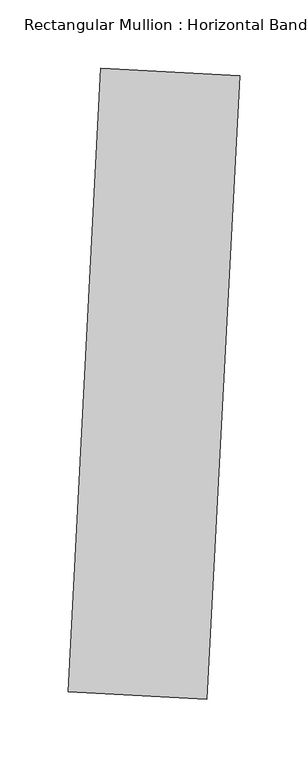
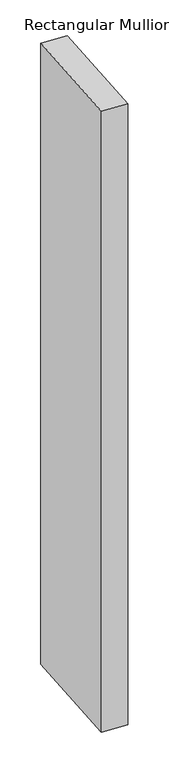
"""IFC4 building model written with IfcOpenShell, lengths in millimetres: member geometry, Rectangular Mullion : Horizontal Band."""

import ifcopenshell
import ifcopenshell.guid

model = None  # the IFC model being written
_history = None  # IfcOwnerHistory: only IFC2X3 demands one
_inside = {}  # id of a spatial element -> (the spatial element, [elements in it])
_under = {}  # id of a project, library or spatial element -> (it, [spatial elements below it])
_declared = {}  # id of a project -> (the project, [libraries it declares])
_typed = {}  # id of a type object -> (the type object, [elements of that type])
_made_of = {}  # id of a material, layer set ... -> (it, [elements and type objects made of it])


def new_model(schema):
    """Start an empty IFC model of exactly this schema.

    Asked for "IFC4X3", IfcOpenShell would pick the latest addendum, in which some entities
    have other attributes; the version numbers below select the first issue.
    IFC2X3 requires an IfcOwnerHistory on every rooted entity: one is made here for all.
    """
    global model, _history
    if schema == "IFC4X3":
        model = ifcopenshell.file(schema_version=(4, 3, 0, 0))
    else:
        model = ifcopenshell.file(schema=schema)
    _inside.clear()
    _under.clear()
    _declared.clear()
    _typed.clear()
    _made_of.clear()
    _history = None
    if model.schema == "IFC2X3":
        org = make("IfcOrganization", Name="unknown")
        user = make(
            "IfcPersonAndOrganization",
            ThePerson=make("IfcPerson", FamilyName="unknown"),
            TheOrganization=org,
        )
        app = make(
            "IfcApplication",
            ApplicationDeveloper=org,
            Version="unknown",
            ApplicationFullName="unknown",
            ApplicationIdentifier="unknown",
        )
        _history = make(
            "IfcOwnerHistory",
            OwningUser=user,
            OwningApplication=app,
            ChangeAction="ADDED",
            CreationDate=0,
        )
    return model


def make(cls, **values):
    """One entity of the class cls with the attributes given. An attribute that is None is left unset."""
    return model.create_entity(
        cls, **{name: value for name, value in values.items() if value is not None}
    )


def rooted(cls, **values):
    """An entity with a GlobalId (a new one), such as an element, a storey or a relation."""
    return make(cls, GlobalId=ifcopenshell.guid.new(), OwnerHistory=_history, **values)


def si_unit(unit_type, name, prefix=None):
    """IfcSIUnit, for example si_unit("LENGTHUNIT", "METRE", prefix="MILLI")."""
    return make("IfcSIUnit", UnitType=unit_type, Prefix=prefix, Name=name)


def assignment(units):
    """IfcUnitAssignment: the units of a project."""
    return None if units is None else make("IfcUnitAssignment", Units=units)


def point(xyz):
    """IfcCartesianPoint."""
    return None if xyz is None else make("IfcCartesianPoint", Coordinates=xyz)


def direction(xyz):
    """IfcDirection."""
    return None if xyz is None else make("IfcDirection", DirectionRatios=xyz)


def frame(location, z_axis=None, x_axis=None):
    """IfcAxis2Placement3D, a coordinate frame: its origin and axes. An axis left out is left unset."""
    return make(
        "IfcAxis2Placement3D",
        Location=point(location),
        Axis=direction(z_axis),
        RefDirection=direction(x_axis),
    )


def origin():
    """The frame at (0, 0, 0) with its axes left unset."""
    return frame((0.0, 0.0, 0.0))


def place(relative_to, where):
    """IfcLocalPlacement: puts the frame where relative to a parent placement (None: the world)."""
    return make(
        "IfcLocalPlacement", PlacementRelTo=relative_to, RelativePlacement=where
    )


def context(
    kind, dimensions, precision=None, world=None, true_north=None, identifier=None
):
    """IfcGeometricRepresentationContext, for example the 3D "Model" context."""
    return make(
        "IfcGeometricRepresentationContext",
        ContextIdentifier=identifier,
        ContextType=kind,
        CoordinateSpaceDimension=dimensions,
        Precision=precision,
        WorldCoordinateSystem=world,
        TrueNorth=true_north,
    )


def project(units=None, contexts=None):
    """IfcProject with its units and contexts."""
    return rooted(
        "IfcProject",
        Name="project",
        RepresentationContexts=contexts,
        UnitsInContext=assignment(units),
    )


def spatial(cls, under=None, at=None, **own):
    """A site, building, storey or space (cls), placed at a placement, below another one or the project."""
    s = rooted(cls, ObjectPlacement=at, **own)
    if under is not None:
        _under.setdefault(under.id(), (under, []))[1].append(s)
    return s


def polyline(points):
    """IfcPolyline through the points."""
    return make("IfcPolyline", Points=[point(p) for p in points])


def outline(outer, holes=None, kind="AREA"):
    """IfcArbitraryClosedProfileDef: a profile drawn as a closed curve; with holes, ...WithVoids."""
    if holes is None:
        return make("IfcArbitraryClosedProfileDef", ProfileType=kind, OuterCurve=outer)
    return make(
        "IfcArbitraryProfileDefWithVoids",
        ProfileType=kind,
        OuterCurve=outer,
        InnerCurves=holes,
    )


def extrude(swept, where, along, depth):
    """IfcExtrudedAreaSolid: the profile swept, set in the frame where, extruded along a direction by depth."""
    return make(
        "IfcExtrudedAreaSolid",
        SweptArea=swept,
        Position=where,
        ExtrudedDirection=direction(along),
        Depth=depth,
    )


def shape(context_of_items, identifier, shape_type, items):
    """IfcShapeRepresentation: the items that make up one representation, for example the "Body"."""
    return make(
        "IfcShapeRepresentation",
        ContextOfItems=context_of_items,
        RepresentationIdentifier=identifier,
        RepresentationType=shape_type,
        Items=items,
    )


def source(mapping_origin, context_of_items, identifier, shape_type, items):
    """IfcRepresentationMap: a shape defined once, which mapped items show again and again."""
    return make(
        "IfcRepresentationMap",
        MappingOrigin=mapping_origin,
        MappedRepresentation=shape(context_of_items, identifier, shape_type, items),
    )


def transform(
    local_origin,
    x_axis=None,
    y_axis=None,
    z_axis=None,
    scale=None,
    scale2=None,
    scale3=None,
    uniform=True,
):
    """IfcCartesianTransformationOperator3D, or its non-uniform kind. x_axis, y_axis, z_axis: its Axis1, 2, 3."""
    if uniform:
        return make(
            "IfcCartesianTransformationOperator3D",
            Axis1=direction(x_axis),
            Axis2=direction(y_axis),
            LocalOrigin=point(local_origin),
            Scale=scale,
            Axis3=direction(z_axis),
        )
    return make(
        "IfcCartesianTransformationOperator3DnonUniform",
        Axis1=direction(x_axis),
        Axis2=direction(y_axis),
        LocalOrigin=point(local_origin),
        Scale=scale,
        Axis3=direction(z_axis),
        Scale2=scale2,
        Scale3=scale3,
    )


def mapped(mapping_source, mapping_target):
    """IfcMappedItem: shows the shape of a source again, moved by a transform."""
    return make(
        "IfcMappedItem", MappingSource=mapping_source, MappingTarget=mapping_target
    )


def made_of(thing, what):
    """Note that an element or type object is made of a material, layer set ...; save() writes the relation."""
    if what is not None:
        _made_of.setdefault(what.id(), (what, []))[1].append(thing)
    return thing


def element(
    cls,
    number,
    at=None,
    inside=None,
    cuts=None,
    type_object=None,
    material=None,
    context=None,
    identifier="Body",
    shape_type=None,
    held_by="IfcProductDefinitionShape",
    body=None,
    shapes=None,
    **own,
):
    """One element of the class cls, such as IfcWall. Its Tag is "e" and its number.

    at: its placement. inside: the storey or other place that contains it. cuts: it is an
    opening in that element (IfcRelVoidsElement). A single representation is given by context,
    identifier, shape_type and body (its items); several are given by shapes. held_by: the class
    of the entity that holds the representations. save() writes the other relations.
    """
    e = rooted(cls, Tag="e%d" % number, ObjectPlacement=at, **own)
    if body is not None:
        shapes = [shape(context, identifier, shape_type, body)]
    if shapes is not None:
        e.Representation = make(held_by, Representations=shapes)
    if inside is not None:
        _inside.setdefault(inside.id(), (inside, []))[1].append(e)
    if cuts is not None:
        rooted(
            "IfcRelVoidsElement", RelatingBuildingElement=cuts, RelatedOpeningElement=e
        )
    if type_object is not None:
        _typed.setdefault(type_object.id(), (type_object, []))[1].append(e)
    return made_of(e, material)


def aggregate(whole, parts):
    """IfcRelAggregates: a whole, such as a stair, and the parts it consists of."""
    return rooted("IfcRelAggregates", RelatingObject=whole, RelatedObjects=parts)


def save(model, path):
    """Write the relations noted so far, then the file.

    IfcRelAggregates (storeys below a building ...), IfcRelContainedInSpatialStructure (elements
    in a storey), IfcRelDefinesByType, IfcRelAssociatesMaterial and IfcRelDeclares: one each for
    every whole, place, type object, material and project.
    """
    for whole, parts in _under.values():
        aggregate(whole, parts)
    for where, things in _inside.values():
        rooted(
            "IfcRelContainedInSpatialStructure",
            RelatedElements=things,
            RelatingStructure=where,
        )
    for kind, things in _typed.values():
        rooted("IfcRelDefinesByType", RelatedObjects=things, RelatingType=kind)
    for what, things in _made_of.values():
        rooted("IfcRelAssociatesMaterial", RelatedObjects=things, RelatingMaterial=what)
    for by, libraries in _declared.values():
        rooted("IfcRelDeclares", RelatingContext=by, RelatedDefinitions=libraries)
    model.write(path)


def rectangular_mullion_horizontal_band_838d4356(model_context):
    return source(origin(), model_context, "Body", "SweptSolid", [
        extrude(outline(polyline([(62.69438, 301.8280451), (38.7663808, -154.7453782), (-62.69438, -149.4280451), (-38.7663808, 307.1453782), (62.69438, 301.8280451)])), frame((0.0, 0.0, -2603.6943143), z_axis=(0.0, 0.0, 1.0), x_axis=(1.0, 0.0, 0.0)), (0.0, 0.0, 1.0), 2603.6943143),
    ])


if __name__ == "__main__":
    model = new_model("IFC4")
    model_context = context("Model", 3, world=origin())
    ifc_project = project(units=[si_unit("LENGTHUNIT", "METRE", prefix="MILLI")], contexts=[model_context])
    site = spatial("IfcSite", under=ifc_project)
    building = spatial("IfcBuilding", under=site)
    placement = place(None, origin())
    rectangular_mullion_horizontal_band_shape = rectangular_mullion_horizontal_band_838d4356(model_context)
    element("IfcMember", 1, ObjectType="Rectangular Mullion : Horizontal Band", at=placement, inside=building, context=model_context, shape_type="MappedRepresentation", body=[
        mapped(rectangular_mullion_horizontal_band_shape, transform((0.0, 0.0, 0.0), x_axis=(1.0, 0.0, 0.0), y_axis=(0.0, 1.0, 0.0), z_axis=(0.0, 0.0, 1.0))),
    ])
    save(model, "model.ifc")

# Revit data of these elements
# Type "Rectangular Mullion : Horizontal Band"
#   built-in parameter 1007351 = 0.25 (stored number, unit not read)
#   built-in parameter 1007304 = 1.5 (stored number, unit not read)
#   built-in parameter 1007301 = 0.166667 (stored number, unit not read)
#   built-in parameter 1007300 = 0.166667 (stored number, unit not read)
# Element 1 (IfcMember, "Rectangular Mullion : Horizontal Band")
#   Materials on its faces: "Aluminum"
# Materials
#   "Aluminum": class "Metal", colour RGB 247 247 247, transparency 0, Description = "Aluminum 6061", Cost = 0
